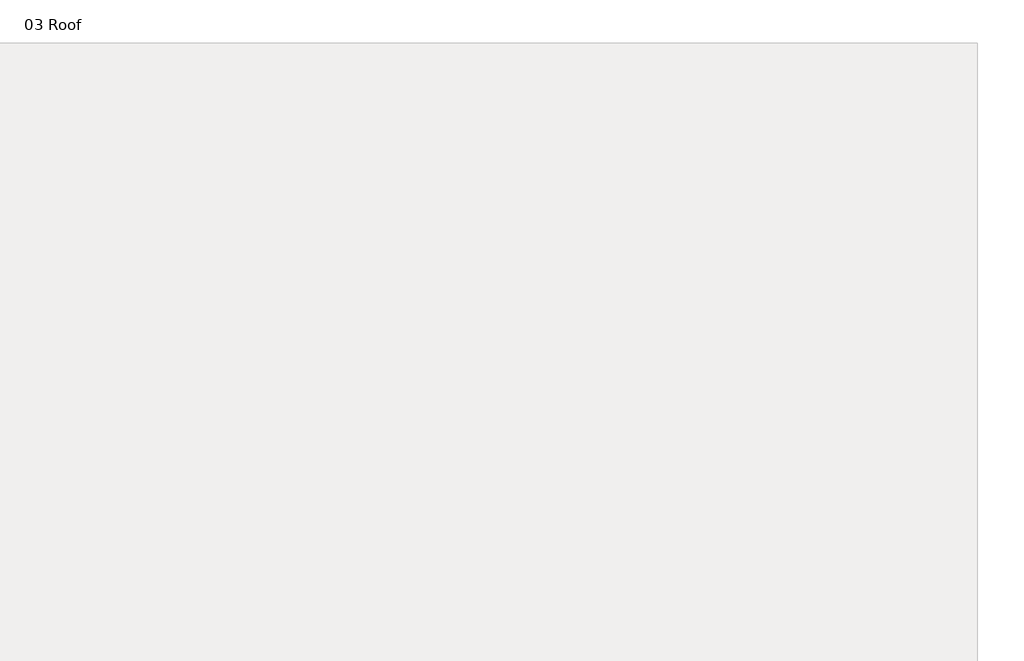
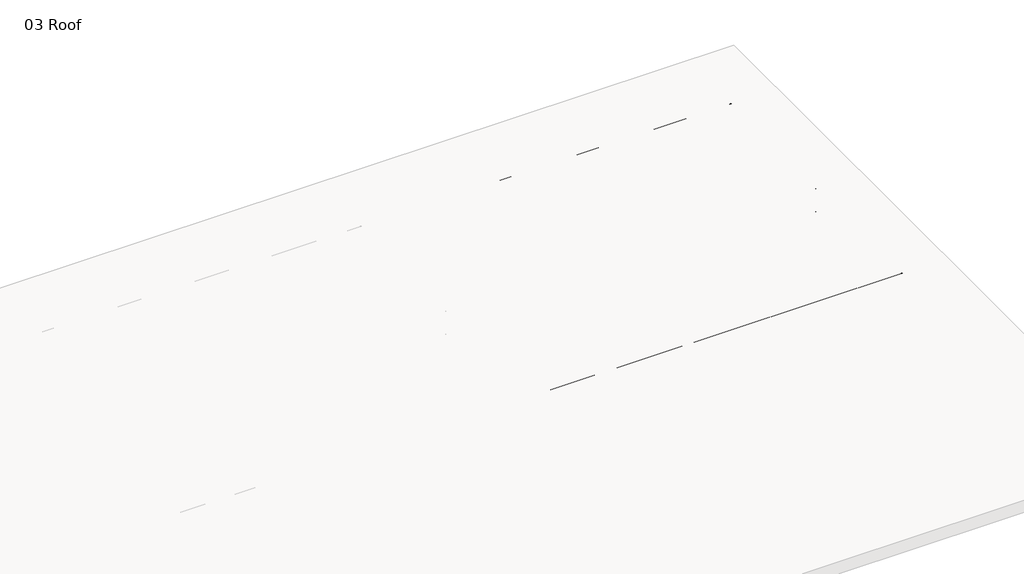
# One storey, part 4 of 4: 102 beams.
"""IFC4 building model written with IfcOpenShell, lengths in millimetres."""

import ifcopenshell
import ifcopenshell.guid

model = None  # the IFC model being written
_history = None  # IfcOwnerHistory: only IFC2X3 demands one
_inside = {}  # id of a spatial element -> (the spatial element, [elements in it])
_under = {}  # id of a project, library or spatial element -> (it, [spatial elements below it])
_declared = {}  # id of a project -> (the project, [libraries it declares])
_typed = {}  # id of a type object -> (the type object, [elements of that type])
_made_of = {}  # id of a material, layer set ... -> (it, [elements and type objects made of it])


def new_model(schema):
    """Start an empty IFC model of exactly this schema.

    Asked for "IFC4X3", IfcOpenShell would pick the latest addendum, in which some entities
    have other attributes; the version numbers below select the first issue.
    IFC2X3 requires an IfcOwnerHistory on every rooted entity: one is made here for all.
    """
    global model, _history
    if schema == "IFC4X3":
        model = ifcopenshell.file(schema_version=(4, 3, 0, 0))
    else:
        model = ifcopenshell.file(schema=schema)
    _inside.clear()
    _under.clear()
    _declared.clear()
    _typed.clear()
    _made_of.clear()
    _history = None
    if model.schema == "IFC2X3":
        org = make("IfcOrganization", Name="unknown")
        user = make(
            "IfcPersonAndOrganization",
            ThePerson=make("IfcPerson", FamilyName="unknown"),
            TheOrganization=org,
        )
        app = make(
            "IfcApplication",
            ApplicationDeveloper=org,
            Version="unknown",
            ApplicationFullName="unknown",
            ApplicationIdentifier="unknown",
        )
        _history = make(
            "IfcOwnerHistory",
            OwningUser=user,
            OwningApplication=app,
            ChangeAction="ADDED",
            CreationDate=0,
        )
    return model


def make(cls, **values):
    """One entity of the class cls with the attributes given. An attribute that is None is left unset."""
    return model.create_entity(
        cls, **{name: value for name, value in values.items() if value is not None}
    )


def rooted(cls, **values):
    """An entity with a GlobalId (a new one), such as an element, a storey or a relation."""
    return make(cls, GlobalId=ifcopenshell.guid.new(), OwnerHistory=_history, **values)


def si_unit(unit_type, name, prefix=None):
    """IfcSIUnit, for example si_unit("LENGTHUNIT", "METRE", prefix="MILLI")."""
    return make("IfcSIUnit", UnitType=unit_type, Prefix=prefix, Name=name)


def assignment(units):
    """IfcUnitAssignment: the units of a project."""
    return None if units is None else make("IfcUnitAssignment", Units=units)


def point(xyz):
    """IfcCartesianPoint."""
    return None if xyz is None else make("IfcCartesianPoint", Coordinates=xyz)


def direction(xyz):
    """IfcDirection."""
    return None if xyz is None else make("IfcDirection", DirectionRatios=xyz)


def frame(location, z_axis=None, x_axis=None):
    """IfcAxis2Placement3D, a coordinate frame: its origin and axes. An axis left out is left unset."""
    return make(
        "IfcAxis2Placement3D",
        Location=point(location),
        Axis=direction(z_axis),
        RefDirection=direction(x_axis),
    )


def frame_2d(location, x_axis=None):
    """IfcAxis2Placement2D, a coordinate frame in the plane: its origin and x axis."""
    return make(
        "IfcAxis2Placement2D", Location=point(location), RefDirection=direction(x_axis)
    )


def origin():
    """The frame at (0, 0, 0) with its axes left unset."""
    return frame((0.0, 0.0, 0.0))


def place(relative_to, where):
    """IfcLocalPlacement: puts the frame where relative to a parent placement (None: the world)."""
    return make(
        "IfcLocalPlacement", PlacementRelTo=relative_to, RelativePlacement=where
    )


def context(
    kind, dimensions, precision=None, world=None, true_north=None, identifier=None
):
    """IfcGeometricRepresentationContext, for example the 3D "Model" context."""
    return make(
        "IfcGeometricRepresentationContext",
        ContextIdentifier=identifier,
        ContextType=kind,
        CoordinateSpaceDimension=dimensions,
        Precision=precision,
        WorldCoordinateSystem=world,
        TrueNorth=true_north,
    )


def project(units=None, contexts=None):
    """IfcProject with its units and contexts."""
    return rooted(
        "IfcProject",
        Name="project",
        RepresentationContexts=contexts,
        UnitsInContext=assignment(units),
    )


def spatial(cls, under=None, at=None, **own):
    """A site, building, storey or space (cls), placed at a placement, below another one or the project."""
    s = rooted(cls, ObjectPlacement=at, **own)
    if under is not None:
        _under.setdefault(under.id(), (under, []))[1].append(s)
    return s


def polyline(points):
    """IfcPolyline through the points."""
    return make("IfcPolyline", Points=[point(p) for p in points])


def circle_curve(where, radius):
    """IfcCircle in the frame where."""
    return make("IfcCircle", Position=where, Radius=radius)


def trimmed(basis, trim1, trim2, sense, master):
    """IfcTrimmedCurve: the piece of a basis curve between two trims."""
    return make(
        "IfcTrimmedCurve",
        BasisCurve=basis,
        Trim1=trim1,
        Trim2=trim2,
        SenseAgreement=sense,
        MasterRepresentation=master,
    )


def segment(curve, same_sense, transition):
    """IfcCompositeCurveSegment."""
    return make(
        "IfcCompositeCurveSegment",
        Transition=transition,
        SameSense=same_sense,
        ParentCurve=curve,
    )


def composite_curve(segments, self_intersect=None):
    """IfcCompositeCurve: segments joined end to end."""
    return make("IfcCompositeCurve", Segments=segments, SelfIntersect=self_intersect)


def outline(outer, holes=None, kind="AREA"):
    """IfcArbitraryClosedProfileDef: a profile drawn as a closed curve; with holes, ...WithVoids."""
    if holes is None:
        return make("IfcArbitraryClosedProfileDef", ProfileType=kind, OuterCurve=outer)
    return make(
        "IfcArbitraryProfileDefWithVoids",
        ProfileType=kind,
        OuterCurve=outer,
        InnerCurves=holes,
    )


def extrude(swept, where, along, depth):
    """IfcExtrudedAreaSolid: the profile swept, set in the frame where, extruded along a direction by depth."""
    return make(
        "IfcExtrudedAreaSolid",
        SweptArea=swept,
        Position=where,
        ExtrudedDirection=direction(along),
        Depth=depth,
    )


def shape(context_of_items, identifier, shape_type, items):
    """IfcShapeRepresentation: the items that make up one representation, for example the "Body"."""
    return make(
        "IfcShapeRepresentation",
        ContextOfItems=context_of_items,
        RepresentationIdentifier=identifier,
        RepresentationType=shape_type,
        Items=items,
    )


def source(mapping_origin, context_of_items, identifier, shape_type, items):
    """IfcRepresentationMap: a shape defined once, which mapped items show again and again."""
    return make(
        "IfcRepresentationMap",
        MappingOrigin=mapping_origin,
        MappedRepresentation=shape(context_of_items, identifier, shape_type, items),
    )


def transform(
    local_origin,
    x_axis=None,
    y_axis=None,
    z_axis=None,
    scale=None,
    scale2=None,
    scale3=None,
    uniform=True,
):
    """IfcCartesianTransformationOperator3D, or its non-uniform kind. x_axis, y_axis, z_axis: its Axis1, 2, 3."""
    if uniform:
        return make(
            "IfcCartesianTransformationOperator3D",
            Axis1=direction(x_axis),
            Axis2=direction(y_axis),
            LocalOrigin=point(local_origin),
            Scale=scale,
            Axis3=direction(z_axis),
        )
    return make(
        "IfcCartesianTransformationOperator3DnonUniform",
        Axis1=direction(x_axis),
        Axis2=direction(y_axis),
        LocalOrigin=point(local_origin),
        Scale=scale,
        Axis3=direction(z_axis),
        Scale2=scale2,
        Scale3=scale3,
    )


def mapped(mapping_source, mapping_target):
    """IfcMappedItem: shows the shape of a source again, moved by a transform."""
    return make(
        "IfcMappedItem", MappingSource=mapping_source, MappingTarget=mapping_target
    )


def made_of(thing, what):
    """Note that an element or type object is made of a material, layer set ...; save() writes the relation."""
    if what is not None:
        _made_of.setdefault(what.id(), (what, []))[1].append(thing)
    return thing


def element(
    cls,
    number,
    at=None,
    inside=None,
    cuts=None,
    type_object=None,
    material=None,
    context=None,
    identifier="Body",
    shape_type=None,
    held_by="IfcProductDefinitionShape",
    body=None,
    shapes=None,
    **own,
):
    """One element of the class cls, such as IfcWall. Its Tag is "e" and its number.

    at: its placement. inside: the storey or other place that contains it. cuts: it is an
    opening in that element (IfcRelVoidsElement). A single representation is given by context,
    identifier, shape_type and body (its items); several are given by shapes. held_by: the class
    of the entity that holds the representations. save() writes the other relations.
    """
    e = rooted(cls, Tag="e%d" % number, ObjectPlacement=at, **own)
    if body is not None:
        shapes = [shape(context, identifier, shape_type, body)]
    if shapes is not None:
        e.Representation = make(held_by, Representations=shapes)
    if inside is not None:
        _inside.setdefault(inside.id(), (inside, []))[1].append(e)
    if cuts is not None:
        rooted(
            "IfcRelVoidsElement", RelatingBuildingElement=cuts, RelatedOpeningElement=e
        )
    if type_object is not None:
        _typed.setdefault(type_object.id(), (type_object, []))[1].append(e)
    return made_of(e, material)


def aggregate(whole, parts):
    """IfcRelAggregates: a whole, such as a stair, and the parts it consists of."""
    return rooted("IfcRelAggregates", RelatingObject=whole, RelatedObjects=parts)


def save(model, path):
    """Write the relations noted so far, then the file.

    IfcRelAggregates (storeys below a building ...), IfcRelContainedInSpatialStructure (elements
    in a storey), IfcRelDefinesByType, IfcRelAssociatesMaterial and IfcRelDeclares: one each for
    every whole, place, type object, material and project.
    """
    for whole, parts in _under.values():
        aggregate(whole, parts)
    for where, things in _inside.values():
        rooted(
            "IfcRelContainedInSpatialStructure",
            RelatedElements=things,
            RelatingStructure=where,
        )
    for kind, things in _typed.values():
        rooted("IfcRelDefinesByType", RelatedObjects=things, RelatingType=kind)
    for what, things in _made_of.values():
        rooted("IfcRelAssociatesMaterial", RelatedObjects=things, RelatingMaterial=what)
    for by, libraries in _declared.values():
        rooted("IfcRelDeclares", RelatingContext=by, RelatedDefinitions=libraries)
    model.write(path)


def ub_universal_beam_305x165x40ub_24de31be(model_context):
    return source(origin(), model_context, "Body", "SweptSolid", [
        extrude(outline(composite_curve([segment(polyline([(82.5, -141.5), (82.5, -151.7), (-82.5, -151.7), (-82.5, -141.5), (-11.9, -141.5)]), True, "CONTINUOUS"), segment(trimmed(circle_curve(frame_2d((-11.9, -132.6)), 8.9), [point((-11.9, -141.5))], [point((-3.0, -132.6))], True, "CARTESIAN"), True, "CONTINUOUS"), segment(polyline([(-3.0, -132.6), (-3.0, 132.6)]), True, "CONTINUOUS"), segment(trimmed(circle_curve(frame_2d((-11.9, 132.6)), 8.9), [point((-3.0, 132.6))], [point((-11.9, 141.5))], True, "CARTESIAN"), True, "CONTINUOUS"), segment(polyline([(-11.9, 141.5), (-82.5, 141.5), (-82.5, 151.7), (82.5, 151.7), (82.5, 141.5), (11.9, 141.5)]), True, "CONTINUOUS"), segment(trimmed(circle_curve(frame_2d((11.9, 132.6)), 8.9), [point((11.9, 141.5))], [point((3.0, 132.6))], True, "CARTESIAN"), True, "CONTINUOUS"), segment(polyline([(3.0, 132.6), (3.0, -132.6)]), True, "CONTINUOUS"), segment(trimmed(circle_curve(frame_2d((11.9, -132.6)), 8.9), [point((3.0, -132.6))], [point((11.9, -141.5))], True, "CARTESIAN"), True, "CONTINUOUS"), segment(polyline([(11.9, -141.5), (82.5, -141.5)]), True, "CONTINUOUS")], self_intersect=False)), frame((-335.6, 0.0, 0.0), z_axis=(1.0, 0.0, 0.0), x_axis=(0.0, 1.0, 0.0)), (0.0, 0.0, 1.0), 671.2),
    ])


def ub_universal_beam_305x165x40ub_f67fc52f(model_context):
    return source(origin(), model_context, "Body", "SweptSolid", [
        extrude(outline(composite_curve([segment(polyline([(82.5, -141.5), (82.5, -151.7), (-82.5, -151.7), (-82.5, -141.5), (-11.9, -141.5)]), True, "CONTINUOUS"), segment(trimmed(circle_curve(frame_2d((-11.9, -132.6)), 8.9), [point((-11.9, -141.5))], [point((-3.0, -132.6))], True, "CARTESIAN"), True, "CONTINUOUS"), segment(polyline([(-3.0, -132.6), (-3.0, 132.6)]), True, "CONTINUOUS"), segment(trimmed(circle_curve(frame_2d((-11.9, 132.6)), 8.9), [point((-3.0, 132.6))], [point((-11.9, 141.5))], True, "CARTESIAN"), True, "CONTINUOUS"), segment(polyline([(-11.9, 141.5), (-82.5, 141.5), (-82.5, 151.7), (82.5, 151.7), (82.5, 141.5), (11.9, 141.5)]), True, "CONTINUOUS"), segment(trimmed(circle_curve(frame_2d((11.9, 132.6)), 8.9), [point((11.9, 141.5))], [point((3.0, 132.6))], True, "CARTESIAN"), True, "CONTINUOUS"), segment(polyline([(3.0, 132.6), (3.0, -132.6)]), True, "CONTINUOUS"), segment(trimmed(circle_curve(frame_2d((11.9, -132.6)), 8.9), [point((3.0, -132.6))], [point((11.9, -141.5))], True, "CARTESIAN"), True, "CONTINUOUS"), segment(polyline([(11.9, -141.5), (82.5, -141.5)]), True, "CONTINUOUS")], self_intersect=False)), frame((-7125.0, 0.0, 0.0), z_axis=(1.0, 0.0, 0.0), x_axis=(0.0, 1.0, 0.0)), (0.0, 0.0, 1.0), 14250.0),
    ])


def ub_universal_beam_305x165x40ub_26fb8d3a(model_context):
    return source(origin(), model_context, "Body", "SweptSolid", [
        extrude(outline(composite_curve([segment(polyline([(82.5, -141.5), (82.5, -151.7), (-82.5, -151.7), (-82.5, -141.5), (-11.9, -141.5)]), True, "CONTINUOUS"), segment(trimmed(circle_curve(frame_2d((-11.9, -132.6)), 8.9), [point((-11.9, -141.5))], [point((-3.0, -132.6))], True, "CARTESIAN"), True, "CONTINUOUS"), segment(polyline([(-3.0, -132.6), (-3.0, 132.6)]), True, "CONTINUOUS"), segment(trimmed(circle_curve(frame_2d((-11.9, 132.6)), 8.9), [point((-3.0, 132.6))], [point((-11.9, 141.5))], True, "CARTESIAN"), True, "CONTINUOUS"), segment(polyline([(-11.9, 141.5), (-82.5, 141.5), (-82.5, 151.7), (82.5, 151.7), (82.5, 141.5), (11.9, 141.5)]), True, "CONTINUOUS"), segment(trimmed(circle_curve(frame_2d((11.9, 132.6)), 8.9), [point((11.9, 141.5))], [point((3.0, 132.6))], True, "CARTESIAN"), True, "CONTINUOUS"), segment(polyline([(3.0, 132.6), (3.0, -132.6)]), True, "CONTINUOUS"), segment(trimmed(circle_curve(frame_2d((11.9, -132.6)), 8.9), [point((3.0, -132.6))], [point((11.9, -141.5))], True, "CARTESIAN"), True, "CONTINUOUS"), segment(polyline([(11.9, -141.5), (82.5, -141.5)]), True, "CONTINUOUS")], self_intersect=False)), frame((-347.8807825, 0.0, 0.0), z_axis=(1.0, 0.0, 0.0), x_axis=(0.0, 1.0, 0.0)), (0.0, 0.0, 1.0), 695.761565),
    ])


model = new_model("IFC4")

# Units and contexts
model_context = context("Model", 3, world=origin())
ifc_project = project(units=[si_unit("LENGTHUNIT", "METRE", prefix="MILLI")], contexts=[model_context])

# Site, building, storey
site = spatial("IfcSite", under=ifc_project)
building = spatial("IfcBuilding", under=site)
storey = spatial("IfcBuildingStorey", under=building, Name="03 Roof", Elevation=8000.0)

# Beams
placement = place(None, origin())
ub_universal_beam_305x165x40ub_shape = ub_universal_beam_305x165x40ub_24de31be(model_context)
element("IfcBeam", 1, ObjectType="UB-Universal Beam : 305x165x40UB", at=placement, inside=storey, context=model_context, shape_type="MappedRepresentation", body=[
    mapped(ub_universal_beam_305x165x40ub_shape, transform((5723.4493174, 12261.9474871, 7500.0), x_axis=(0.0, 0.0, 1.0), y_axis=(0.0, -1.0, 0.0), z_axis=(1.0, 0.0, 0.0))),
])
element("IfcBeam", 2, ObjectType="UB-Universal Beam : 305x165x40UB", at=placement, inside=storey, context=model_context, shape_type="MappedRepresentation", body=[
    mapped(ub_universal_beam_305x165x40ub_shape, transform((4535.9493174, 12261.9474871, 7500.0), x_axis=(0.0, 0.0, 1.0), y_axis=(0.0, -1.0, 0.0), z_axis=(1.0, 0.0, 0.0))),
])
element("IfcBeam", 3, ObjectType="UB-Universal Beam : 305x165x40UB", at=placement, inside=storey, context=model_context, shape_type="MappedRepresentation", body=[
    mapped(ub_universal_beam_305x165x40ub_shape, transform((3348.4493174, 12261.9474871, 7500.0), x_axis=(0.0, 0.0, 1.0), y_axis=(0.0, -1.0, 0.0), z_axis=(1.0, 0.0, 0.0))),
])
element("IfcBeam", 4, ObjectType="UB-Universal Beam : 305x165x40UB", at=placement, inside=storey, context=model_context, shape_type="MappedRepresentation", body=[
    mapped(ub_universal_beam_305x165x40ub_shape, transform((2160.9493174, 12261.9474871, 7500.0), x_axis=(0.0, 0.0, 1.0), y_axis=(0.0, -1.0, 0.0), z_axis=(1.0, 0.0, 0.0))),
])
element("IfcBeam", 5, ObjectType="UB-Universal Beam : 305x165x40UB", at=placement, inside=storey, context=model_context, shape_type="MappedRepresentation", body=[
    mapped(ub_universal_beam_305x165x40ub_shape, transform((6910.9493174, 12261.9474871, 7500.0), x_axis=(0.0, 0.0, 1.0), y_axis=(0.0, -1.0, 0.0), z_axis=(1.0, 0.0, 0.0))),
])
element("IfcBeam", 6, ObjectType="UB-Universal Beam : 305x165x40UB", at=placement, inside=storey, context=model_context, shape_type="MappedRepresentation", body=[
    mapped(ub_universal_beam_305x165x40ub_shape, transform((973.4493174, 12261.9474871, 7500.0), x_axis=(0.0, 0.0, 1.0), y_axis=(0.0, -1.0, 0.0), z_axis=(1.0, 0.0, 0.0))),
])
element("IfcBeam", 7, ObjectType="UB-Universal Beam : 305x165x40UB", at=placement, inside=storey, context=model_context, shape_type="MappedRepresentation", body=[
    mapped(ub_universal_beam_305x165x40ub_shape, transform((20723.4493174, 12261.9474871, 7500.0), x_axis=(0.0, 0.0, 1.0), y_axis=(0.0, -1.0, 0.0), z_axis=(1.0, 0.0, 0.0))),
])
element("IfcBeam", 8, ObjectType="UB-Universal Beam : 305x165x40UB", at=placement, inside=storey, context=model_context, shape_type="MappedRepresentation", body=[
    mapped(ub_universal_beam_305x165x40ub_shape, transform((8848.4493174, 12261.9474871, 7500.0), x_axis=(0.0, 0.0, 1.0), y_axis=(0.0, -1.0, 0.0), z_axis=(1.0, 0.0, 0.0))),
])
element("IfcBeam", 9, ObjectType="UB-Universal Beam : 305x165x40UB", at=placement, inside=storey, context=model_context, shape_type="MappedRepresentation", body=[
    mapped(ub_universal_beam_305x165x40ub_shape, transform((19535.9493174, 12261.9474871, 7500.0), x_axis=(0.0, 0.0, 1.0), y_axis=(0.0, -1.0, 0.0), z_axis=(1.0, 0.0, 0.0))),
])
element("IfcBeam", 10, ObjectType="UB-Universal Beam : 305x165x40UB", at=placement, inside=storey, context=model_context, shape_type="MappedRepresentation", body=[
    mapped(ub_universal_beam_305x165x40ub_shape, transform((10035.9493174, 12261.9474871, 7500.0), x_axis=(0.0, 0.0, 1.0), y_axis=(0.0, -1.0, 0.0), z_axis=(1.0, 0.0, 0.0))),
])
element("IfcBeam", 11, ObjectType="UB-Universal Beam : 305x165x40UB", at=placement, inside=storey, context=model_context, shape_type="MappedRepresentation", body=[
    mapped(ub_universal_beam_305x165x40ub_shape, transform((18348.4493174, 12261.9474871, 7500.0), x_axis=(0.0, 0.0, 1.0), y_axis=(0.0, -1.0, 0.0), z_axis=(1.0, 0.0, 0.0))),
])
element("IfcBeam", 12, ObjectType="UB-Universal Beam : 305x165x40UB", at=placement, inside=storey, context=model_context, shape_type="MappedRepresentation", body=[
    mapped(ub_universal_beam_305x165x40ub_shape, transform((17160.9493174, 12261.9474871, 7500.0), x_axis=(0.0, 0.0, 1.0), y_axis=(0.0, -1.0, 0.0), z_axis=(1.0, 0.0, 0.0))),
])
element("IfcBeam", 13, ObjectType="UB-Universal Beam : 305x165x40UB", at=placement, inside=storey, context=model_context, shape_type="MappedRepresentation", body=[
    mapped(ub_universal_beam_305x165x40ub_shape, transform((21910.9493174, 12261.9474871, 7500.0), x_axis=(0.0, 0.0, 1.0), y_axis=(0.0, -1.0, 0.0), z_axis=(1.0, 0.0, 0.0))),
])
element("IfcBeam", 14, ObjectType="UB-Universal Beam : 305x165x40UB", at=placement, inside=storey, context=model_context, shape_type="MappedRepresentation", body=[
    mapped(ub_universal_beam_305x165x40ub_shape, transform((15973.4493174, 12261.9474871, 7500.0), x_axis=(0.0, 0.0, 1.0), y_axis=(0.0, -1.0, 0.0), z_axis=(1.0, 0.0, 0.0))),
])
element("IfcBeam", 15, ObjectType="UB-Universal Beam : 305x165x40UB", at=placement, inside=storey, context=model_context, shape_type="MappedRepresentation", body=[
    mapped(ub_universal_beam_305x165x40ub_shape, transform((11223.4493174, 12261.9474871, 7500.0), x_axis=(0.0, 0.0, 1.0), y_axis=(0.0, -1.0, 0.0), z_axis=(1.0, 0.0, 0.0))),
])
element("IfcBeam", 16, ObjectType="UB-Universal Beam : 305x165x40UB", at=placement, inside=storey, context=model_context, shape_type="MappedRepresentation", body=[
    mapped(ub_universal_beam_305x165x40ub_shape, transform((12410.9493174, 12261.9474871, 7500.0), x_axis=(0.0, 0.0, 1.0), y_axis=(0.0, -1.0, 0.0), z_axis=(1.0, 0.0, 0.0))),
])
element("IfcBeam", 17, ObjectType="UB-Universal Beam : 305x165x40UB", at=placement, inside=storey, context=model_context, shape_type="MappedRepresentation", body=[
    mapped(ub_universal_beam_305x165x40ub_shape, transform((7660.9493174, 12261.9474871, 7500.0), x_axis=(0.0, 0.0, 1.0), y_axis=(0.0, -1.0, 0.0), z_axis=(1.0, 0.0, 0.0))),
])
element("IfcBeam", 18, ObjectType="UB-Universal Beam : 305x165x40UB", at=placement, inside=storey, context=model_context, shape_type="MappedRepresentation", body=[
    mapped(ub_universal_beam_305x165x40ub_shape, transform((13598.4493174, 12261.9474871, 7500.0), x_axis=(0.0, 0.0, 1.0), y_axis=(0.0, -1.0, 0.0), z_axis=(1.0, 0.0, 0.0))),
])
element("IfcBeam", 19, ObjectType="UB-Universal Beam : 305x165x40UB", at=placement, inside=storey, context=model_context, shape_type="MappedRepresentation", body=[
    mapped(ub_universal_beam_305x165x40ub_shape, transform((14785.9493174, 12261.9474871, 7500.0), x_axis=(0.0, 0.0, 1.0), y_axis=(0.0, -1.0, 0.0), z_axis=(1.0, 0.0, 0.0))),
])
element("IfcBeam", 20, ObjectType="UB-Universal Beam : 305x165x40UB", at=placement, inside=storey, context=model_context, shape_type="MappedRepresentation", body=[
    mapped(ub_universal_beam_305x165x40ub_shape, transform((5723.4493174, 6271.8474871, 7500.0), x_axis=(0.0, 0.0, 1.0), y_axis=(0.0, -1.0, 0.0), z_axis=(1.0, 0.0, 0.0))),
])
element("IfcBeam", 21, ObjectType="UB-Universal Beam : 305x165x40UB", at=placement, inside=storey, context=model_context, shape_type="MappedRepresentation", body=[
    mapped(ub_universal_beam_305x165x40ub_shape, transform((4535.9493174, 6271.8474871, 7500.0), x_axis=(0.0, 0.0, 1.0), y_axis=(0.0, -1.0, 0.0), z_axis=(1.0, 0.0, 0.0))),
])
element("IfcBeam", 22, ObjectType="UB-Universal Beam : 305x165x40UB", at=placement, inside=storey, context=model_context, shape_type="MappedRepresentation", body=[
    mapped(ub_universal_beam_305x165x40ub_shape, transform((3348.4493174, 6271.8474871, 7500.0), x_axis=(0.0, 0.0, 1.0), y_axis=(0.0, -1.0, 0.0), z_axis=(1.0, 0.0, 0.0))),
])
element("IfcBeam", 23, ObjectType="UB-Universal Beam : 305x165x40UB", at=placement, inside=storey, context=model_context, shape_type="MappedRepresentation", body=[
    mapped(ub_universal_beam_305x165x40ub_shape, transform((2160.9493174, 6271.8474871, 7500.0), x_axis=(0.0, 0.0, 1.0), y_axis=(0.0, -1.0, 0.0), z_axis=(1.0, 0.0, 0.0))),
])
element("IfcBeam", 24, ObjectType="UB-Universal Beam : 305x165x40UB", at=placement, inside=storey, context=model_context, shape_type="MappedRepresentation", body=[
    mapped(ub_universal_beam_305x165x40ub_shape, transform((6910.9493174, 6271.8474871, 7500.0), x_axis=(0.0, 0.0, 1.0), y_axis=(0.0, -1.0, 0.0), z_axis=(1.0, 0.0, 0.0))),
])
element("IfcBeam", 25, ObjectType="UB-Universal Beam : 305x165x40UB", at=placement, inside=storey, context=model_context, shape_type="MappedRepresentation", body=[
    mapped(ub_universal_beam_305x165x40ub_shape, transform((20723.4493174, 6271.8474871, 7500.0), x_axis=(0.0, 0.0, 1.0), y_axis=(0.0, -1.0, 0.0), z_axis=(1.0, 0.0, 0.0))),
])
element("IfcBeam", 26, ObjectType="UB-Universal Beam : 305x165x40UB", at=placement, inside=storey, context=model_context, shape_type="MappedRepresentation", body=[
    mapped(ub_universal_beam_305x165x40ub_shape, transform((8848.4493174, 6271.8474871, 7500.0), x_axis=(0.0, 0.0, 1.0), y_axis=(0.0, -1.0, 0.0), z_axis=(1.0, 0.0, 0.0))),
])
element("IfcBeam", 27, ObjectType="UB-Universal Beam : 305x165x40UB", at=placement, inside=storey, context=model_context, shape_type="MappedRepresentation", body=[
    mapped(ub_universal_beam_305x165x40ub_shape, transform((19535.9493174, 6271.8474871, 7500.0), x_axis=(0.0, 0.0, 1.0), y_axis=(0.0, -1.0, 0.0), z_axis=(1.0, 0.0, 0.0))),
])
element("IfcBeam", 28, ObjectType="UB-Universal Beam : 305x165x40UB", at=placement, inside=storey, context=model_context, shape_type="MappedRepresentation", body=[
    mapped(ub_universal_beam_305x165x40ub_shape, transform((10035.9493174, 6271.8474871, 7500.0), x_axis=(0.0, 0.0, 1.0), y_axis=(0.0, -1.0, 0.0), z_axis=(1.0, 0.0, 0.0))),
])
element("IfcBeam", 29, ObjectType="UB-Universal Beam : 305x165x40UB", at=placement, inside=storey, context=model_context, shape_type="MappedRepresentation", body=[
    mapped(ub_universal_beam_305x165x40ub_shape, transform((18348.4493174, 6271.8474871, 7500.0), x_axis=(0.0, 0.0, 1.0), y_axis=(0.0, -1.0, 0.0), z_axis=(1.0, 0.0, 0.0))),
])
element("IfcBeam", 30, ObjectType="UB-Universal Beam : 305x165x40UB", at=placement, inside=storey, context=model_context, shape_type="MappedRepresentation", body=[
    mapped(ub_universal_beam_305x165x40ub_shape, transform((17160.9493174, 6271.8474871, 7500.0), x_axis=(0.0, 0.0, 1.0), y_axis=(0.0, -1.0, 0.0), z_axis=(1.0, 0.0, 0.0))),
])
element("IfcBeam", 31, ObjectType="UB-Universal Beam : 305x165x40UB", at=placement, inside=storey, context=model_context, shape_type="MappedRepresentation", body=[
    mapped(ub_universal_beam_305x165x40ub_shape, transform((21910.9493174, 6271.8474871, 7500.0), x_axis=(0.0, 0.0, 1.0), y_axis=(0.0, -1.0, 0.0), z_axis=(1.0, 0.0, 0.0))),
])
element("IfcBeam", 32, ObjectType="UB-Universal Beam : 305x165x40UB", at=placement, inside=storey, context=model_context, shape_type="MappedRepresentation", body=[
    mapped(ub_universal_beam_305x165x40ub_shape, transform((15973.4493174, 6271.8474871, 7500.0), x_axis=(0.0, 0.0, 1.0), y_axis=(0.0, -1.0, 0.0), z_axis=(1.0, 0.0, 0.0))),
])
element("IfcBeam", 33, ObjectType="UB-Universal Beam : 305x165x40UB", at=placement, inside=storey, context=model_context, shape_type="MappedRepresentation", body=[
    mapped(ub_universal_beam_305x165x40ub_shape, transform((11223.4493174, 6271.8474871, 7500.0), x_axis=(0.0, 0.0, 1.0), y_axis=(0.0, -1.0, 0.0), z_axis=(1.0, 0.0, 0.0))),
])
element("IfcBeam", 34, ObjectType="UB-Universal Beam : 305x165x40UB", at=placement, inside=storey, context=model_context, shape_type="MappedRepresentation", body=[
    mapped(ub_universal_beam_305x165x40ub_shape, transform((12410.9493174, 6271.8474871, 7500.0), x_axis=(0.0, 0.0, 1.0), y_axis=(0.0, -1.0, 0.0), z_axis=(1.0, 0.0, 0.0))),
])
element("IfcBeam", 35, ObjectType="UB-Universal Beam : 305x165x40UB", at=placement, inside=storey, context=model_context, shape_type="MappedRepresentation", body=[
    mapped(ub_universal_beam_305x165x40ub_shape, transform((7660.9493174, 6271.8474871, 7500.0), x_axis=(0.0, 0.0, 1.0), y_axis=(0.0, -1.0, 0.0), z_axis=(1.0, 0.0, 0.0))),
])
element("IfcBeam", 36, ObjectType="UB-Universal Beam : 305x165x40UB", at=placement, inside=storey, context=model_context, shape_type="MappedRepresentation", body=[
    mapped(ub_universal_beam_305x165x40ub_shape, transform((13598.4493174, 6271.8474871, 7500.0), x_axis=(0.0, 0.0, 1.0), y_axis=(0.0, -1.0, 0.0), z_axis=(1.0, 0.0, 0.0))),
])
element("IfcBeam", 37, ObjectType="UB-Universal Beam : 305x165x40UB", at=placement, inside=storey, context=model_context, shape_type="MappedRepresentation", body=[
    mapped(ub_universal_beam_305x165x40ub_shape, transform((14785.9493174, 6271.8474871, 7500.0), x_axis=(0.0, 0.0, 1.0), y_axis=(0.0, -1.0, 0.0), z_axis=(1.0, 0.0, 0.0))),
])
element("IfcBeam", 38, ObjectType="UB-Universal Beam : 305x165x40UB", at=placement, inside=storey, context=model_context, shape_type="MappedRepresentation", body=[
    mapped(ub_universal_beam_305x165x40ub_shape, transform((20723.4493174, 271.8474871, 7500.0), x_axis=(0.0, 0.0, 1.0), y_axis=(0.0, -1.0, 0.0), z_axis=(1.0, 0.0, 0.0))),
])
element("IfcBeam", 39, ObjectType="UB-Universal Beam : 305x165x40UB", at=placement, inside=storey, context=model_context, shape_type="MappedRepresentation", body=[
    mapped(ub_universal_beam_305x165x40ub_shape, transform((8848.4493174, 271.8474871, 7500.0), x_axis=(0.0, 0.0, 1.0), y_axis=(0.0, -1.0, 0.0), z_axis=(1.0, 0.0, 0.0))),
])
element("IfcBeam", 40, ObjectType="UB-Universal Beam : 305x165x40UB", at=placement, inside=storey, context=model_context, shape_type="MappedRepresentation", body=[
    mapped(ub_universal_beam_305x165x40ub_shape, transform((19535.9493174, 271.8474871, 7500.0), x_axis=(0.0, 0.0, 1.0), y_axis=(0.0, -1.0, 0.0), z_axis=(1.0, 0.0, 0.0))),
])
element("IfcBeam", 41, ObjectType="UB-Universal Beam : 305x165x40UB", at=placement, inside=storey, context=model_context, shape_type="MappedRepresentation", body=[
    mapped(ub_universal_beam_305x165x40ub_shape, transform((10035.9493174, 271.8474871, 7500.0), x_axis=(0.0, 0.0, 1.0), y_axis=(0.0, -1.0, 0.0), z_axis=(1.0, 0.0, 0.0))),
])
element("IfcBeam", 42, ObjectType="UB-Universal Beam : 305x165x40UB", at=placement, inside=storey, context=model_context, shape_type="MappedRepresentation", body=[
    mapped(ub_universal_beam_305x165x40ub_shape, transform((18348.4493174, 271.8474871, 7500.0), x_axis=(0.0, 0.0, 1.0), y_axis=(0.0, -1.0, 0.0), z_axis=(1.0, 0.0, 0.0))),
])
element("IfcBeam", 43, ObjectType="UB-Universal Beam : 305x165x40UB", at=placement, inside=storey, context=model_context, shape_type="MappedRepresentation", body=[
    mapped(ub_universal_beam_305x165x40ub_shape, transform((17160.9493174, 271.8474871, 7500.0), x_axis=(0.0, 0.0, 1.0), y_axis=(0.0, -1.0, 0.0), z_axis=(1.0, 0.0, 0.0))),
])
element("IfcBeam", 44, ObjectType="UB-Universal Beam : 305x165x40UB", at=placement, inside=storey, context=model_context, shape_type="MappedRepresentation", body=[
    mapped(ub_universal_beam_305x165x40ub_shape, transform((21910.9493174, 271.8474871, 7500.0), x_axis=(0.0, 0.0, 1.0), y_axis=(0.0, -1.0, 0.0), z_axis=(1.0, 0.0, 0.0))),
])
element("IfcBeam", 45, ObjectType="UB-Universal Beam : 305x165x40UB", at=placement, inside=storey, context=model_context, shape_type="MappedRepresentation", body=[
    mapped(ub_universal_beam_305x165x40ub_shape, transform((15973.4493174, 271.8474871, 7500.0), x_axis=(0.0, 0.0, 1.0), y_axis=(0.0, -1.0, 0.0), z_axis=(1.0, 0.0, 0.0))),
])
element("IfcBeam", 46, ObjectType="UB-Universal Beam : 305x165x40UB", at=placement, inside=storey, context=model_context, shape_type="MappedRepresentation", body=[
    mapped(ub_universal_beam_305x165x40ub_shape, transform((11223.4493174, 271.8474871, 7500.0), x_axis=(0.0, 0.0, 1.0), y_axis=(0.0, -1.0, 0.0), z_axis=(1.0, 0.0, 0.0))),
])
element("IfcBeam", 47, ObjectType="UB-Universal Beam : 305x165x40UB", at=placement, inside=storey, context=model_context, shape_type="MappedRepresentation", body=[
    mapped(ub_universal_beam_305x165x40ub_shape, transform((12410.9493174, 271.8474871, 7500.0), x_axis=(0.0, 0.0, 1.0), y_axis=(0.0, -1.0, 0.0), z_axis=(1.0, 0.0, 0.0))),
])
element("IfcBeam", 48, ObjectType="UB-Universal Beam : 305x165x40UB", at=placement, inside=storey, context=model_context, shape_type="MappedRepresentation", body=[
    mapped(ub_universal_beam_305x165x40ub_shape, transform((13598.4493174, 271.8474871, 7500.0), x_axis=(0.0, 0.0, 1.0), y_axis=(0.0, -1.0, 0.0), z_axis=(1.0, 0.0, 0.0))),
])
element("IfcBeam", 49, ObjectType="UB-Universal Beam : 305x165x40UB", at=placement, inside=storey, context=model_context, shape_type="MappedRepresentation", body=[
    mapped(ub_universal_beam_305x165x40ub_shape, transform((14785.9493174, 271.8474871, 7500.0), x_axis=(0.0, 0.0, 1.0), y_axis=(0.0, -1.0, 0.0), z_axis=(1.0, 0.0, 0.0))),
])
ub_universal_beam_305x165x40ub_2_shape = ub_universal_beam_305x165x40ub_f67fc52f(model_context)
element("IfcBeam", 50, ObjectType="UB-Universal Beam : 305x165x40UB", at=placement, inside=storey, context=model_context, shape_type="MappedRepresentation", body=[
    mapped(ub_universal_beam_305x165x40ub_2_shape, transform((14785.9493174, 12261.9474871, 7000.0), x_axis=(1.0, 0.0, 0.0), y_axis=(0.0, 1.0, 0.0), z_axis=(0.0, 0.0, 1.0))),
])
element("IfcBeam", 51, ObjectType="UB-Universal Beam : 305x165x40UB", at=placement, inside=storey, context=model_context, shape_type="MappedRepresentation", body=[
    mapped(ub_universal_beam_305x165x40ub_2_shape, transform((14785.9493174, 12261.9474871, 8000.0), x_axis=(1.0, 0.0, 0.0), y_axis=(0.0, 1.0, 0.0), z_axis=(0.0, 0.0, 1.0))),
])
element("IfcBeam", 52, ObjectType="UB-Universal Beam : 305x165x40UB", at=placement, inside=storey, context=model_context, shape_type="MappedRepresentation", body=[
    mapped(ub_universal_beam_305x165x40ub_2_shape, transform((14785.9493174, 6271.8474871, 7000.0), x_axis=(1.0, 0.0, 0.0), y_axis=(0.0, 1.0, 0.0), z_axis=(0.0, 0.0, 1.0))),
])
element("IfcBeam", 53, ObjectType="UB-Universal Beam : 305x165x40UB", at=placement, inside=storey, context=model_context, shape_type="MappedRepresentation", body=[
    mapped(ub_universal_beam_305x165x40ub_2_shape, transform((14785.9493174, 6271.8474871, 8000.0), x_axis=(1.0, 0.0, 0.0), y_axis=(0.0, 1.0, 0.0), z_axis=(0.0, 0.0, 1.0))),
])
element("IfcBeam", 54, ObjectType="UB-Universal Beam : 305x165x40UB", at=placement, inside=storey, context=model_context, shape_type="MappedRepresentation", body=[
    mapped(ub_universal_beam_305x165x40ub_2_shape, transform((14785.9493174, 271.8474871, 7000.0), x_axis=(1.0, 0.0, 0.0), y_axis=(0.0, 1.0, 0.0), z_axis=(0.0, 0.0, 1.0))),
])
element("IfcBeam", 55, ObjectType="UB-Universal Beam : 305x165x40UB", at=placement, inside=storey, context=model_context, shape_type="MappedRepresentation", body=[
    mapped(ub_universal_beam_305x165x40ub_2_shape, transform((14785.9493174, 271.8474871, 8000.0), x_axis=(1.0, 0.0, 0.0), y_axis=(0.0, 1.0, 0.0), z_axis=(0.0, 0.0, 1.0))),
])
ub_universal_beam_305x165x40ub_3_shape = ub_universal_beam_305x165x40ub_26fb8d3a(model_context)
element("IfcBeam", 56, ObjectType="UB-Universal Beam : 305x165x40UB", at=placement, inside=storey, context=model_context, shape_type="MappedRepresentation", body=[
    mapped(ub_universal_beam_305x165x40ub_3_shape, transform((5129.6993174, 12261.9474871, 7500.0), x_axis=(0.764911198117045, 0.0, 0.6441357457827868), y_axis=(0.0, -1.0, 0.0), z_axis=(0.6441357457827868, 0.0, -0.764911198117045))),
])
element("IfcBeam", 57, ObjectType="UB-Universal Beam : 305x165x40UB", at=placement, inside=storey, context=model_context, shape_type="MappedRepresentation", body=[
    mapped(ub_universal_beam_305x165x40ub_3_shape, transform((3942.1993174, 12261.9474871, 7500.0), x_axis=(0.7649111981170463, 0.0, 0.6441357457827852), y_axis=(0.0, -1.0, 0.0), z_axis=(0.6441357457827852, 0.0, -0.7649111981170463))),
])
element("IfcBeam", 58, ObjectType="UB-Universal Beam : 305x165x40UB", at=placement, inside=storey, context=model_context, shape_type="MappedRepresentation", body=[
    mapped(ub_universal_beam_305x165x40ub_3_shape, transform((2754.6993174, 12261.9474871, 7500.0), x_axis=(0.7649111981170467, 0.0, 0.6441357457827848), y_axis=(0.0, -1.0, 0.0), z_axis=(0.6441357457827848, 0.0, -0.7649111981170467))),
])
element("IfcBeam", 59, ObjectType="UB-Universal Beam : 305x165x40UB", at=placement, inside=storey, context=model_context, shape_type="MappedRepresentation", body=[
    mapped(ub_universal_beam_305x165x40ub_3_shape, transform((1567.1993174, 12261.9474871, 7500.0), x_axis=(0.7649111981170473, 0.0, 0.6441357457827839), y_axis=(0.0, -1.0, 0.0), z_axis=(0.6441357457827839, 0.0, -0.7649111981170473))),
])
element("IfcBeam", 60, ObjectType="UB-Universal Beam : 305x165x40UB", at=placement, inside=storey, context=model_context, shape_type="MappedRepresentation", body=[
    mapped(ub_universal_beam_305x165x40ub_3_shape, transform((6317.1993174, 12261.9474871, 7500.0), x_axis=(0.7649111981170472, 0.0, 0.6441357457827841), y_axis=(0.0, -1.0, 0.0), z_axis=(0.6441357457827841, 0.0, -0.7649111981170472))),
])
element("IfcBeam", 61, ObjectType="UB-Universal Beam : 305x165x40UB", at=placement, inside=storey, context=model_context, shape_type="MappedRepresentation", body=[
    mapped(ub_universal_beam_305x165x40ub_3_shape, transform((379.6993174, 12261.9474871, 7500.0), x_axis=(0.764911198117048, 0.0, 0.6441357457827831), y_axis=(0.0, -1.0, 0.0), z_axis=(0.6441357457827831, 0.0, -0.764911198117048))),
])
element("IfcBeam", 62, ObjectType="UB-Universal Beam : 305x165x40UB", at=placement, inside=storey, context=model_context, shape_type="MappedRepresentation", body=[
    mapped(ub_universal_beam_305x165x40ub_3_shape, transform((20129.6993174, 12261.9474871, 7500.0), x_axis=(0.764911198117045, 0.0, 0.6441357457827868), y_axis=(0.0, -1.0, 0.0), z_axis=(0.6441357457827868, 0.0, -0.764911198117045))),
])
element("IfcBeam", 63, ObjectType="UB-Universal Beam : 305x165x40UB", at=placement, inside=storey, context=model_context, shape_type="MappedRepresentation", body=[
    mapped(ub_universal_beam_305x165x40ub_3_shape, transform((9442.1993174, 12261.9474871, 7500.0), x_axis=(0.7649111981170519, 0.0, -0.6441357457827785), y_axis=(0.0, -1.0, 0.0), z_axis=(-0.6441357457827785, 0.0, -0.7649111981170519))),
])
element("IfcBeam", 64, ObjectType="UB-Universal Beam : 305x165x40UB", at=placement, inside=storey, context=model_context, shape_type="MappedRepresentation", body=[
    mapped(ub_universal_beam_305x165x40ub_3_shape, transform((18942.1993174, 12261.9474871, 7500.0), x_axis=(0.7649111981170457, 0.0, 0.6441357457827859), y_axis=(0.0, -1.0, 0.0), z_axis=(0.6441357457827859, 0.0, -0.7649111981170457))),
])
element("IfcBeam", 65, ObjectType="UB-Universal Beam : 305x165x40UB", at=placement, inside=storey, context=model_context, shape_type="MappedRepresentation", body=[
    mapped(ub_universal_beam_305x165x40ub_3_shape, transform((10629.6993174, 12261.9474871, 7500.0), x_axis=(0.7649111981170518, 0.0, -0.6441357457827787), y_axis=(0.0, -1.0, 0.0), z_axis=(-0.6441357457827787, 0.0, -0.7649111981170518))),
])
element("IfcBeam", 66, ObjectType="UB-Universal Beam : 305x165x40UB", at=placement, inside=storey, context=model_context, shape_type="MappedRepresentation", body=[
    mapped(ub_universal_beam_305x165x40ub_3_shape, transform((17754.6993174, 12261.9474871, 7500.0), x_axis=(0.764911198117047, 0.0, 0.6441357457827844), y_axis=(0.0, -1.0, 0.0), z_axis=(0.6441357457827844, 0.0, -0.764911198117047))),
])
element("IfcBeam", 67, ObjectType="UB-Universal Beam : 305x165x40UB", at=placement, inside=storey, context=model_context, shape_type="MappedRepresentation", body=[
    mapped(ub_universal_beam_305x165x40ub_3_shape, transform((16567.1993174, 12261.9474871, 7500.0), x_axis=(0.764911198117047, 0.0, 0.6441357457827842), y_axis=(0.0, -1.0, 0.0), z_axis=(0.6441357457827842, 0.0, -0.764911198117047))),
])
element("IfcBeam", 68, ObjectType="UB-Universal Beam : 305x165x40UB", at=placement, inside=storey, context=model_context, shape_type="MappedRepresentation", body=[
    mapped(ub_universal_beam_305x165x40ub_3_shape, transform((21317.1993174, 12261.9474871, 7500.0), x_axis=(0.7649111981170478, 0.0, 0.6441357457827834), y_axis=(0.0, -1.0, 0.0), z_axis=(0.6441357457827834, 0.0, -0.7649111981170478))),
])
element("IfcBeam", 69, ObjectType="UB-Universal Beam : 305x165x40UB", at=placement, inside=storey, context=model_context, shape_type="MappedRepresentation", body=[
    mapped(ub_universal_beam_305x165x40ub_3_shape, transform((15379.6993174, 12261.9474871, 7500.0), x_axis=(0.7649111981170477, 0.0, 0.6441357457827834), y_axis=(0.0, -1.0, 0.0), z_axis=(0.6441357457827834, 0.0, -0.7649111981170477))),
])
element("IfcBeam", 70, ObjectType="UB-Universal Beam : 305x165x40UB", at=placement, inside=storey, context=model_context, shape_type="MappedRepresentation", body=[
    mapped(ub_universal_beam_305x165x40ub_3_shape, transform((11817.1993174, 12261.9474871, 7500.0), x_axis=(0.7649111981170504, 0.0, -0.6441357457827802), y_axis=(0.0, -1.0, 0.0), z_axis=(-0.6441357457827802, 0.0, -0.7649111981170504))),
])
element("IfcBeam", 71, ObjectType="UB-Universal Beam : 305x165x40UB", at=placement, inside=storey, context=model_context, shape_type="MappedRepresentation", body=[
    mapped(ub_universal_beam_305x165x40ub_3_shape, transform((13004.6993174, 12261.9474871, 7500.0), x_axis=(0.764911198117051, 0.0, -0.6441357457827797), y_axis=(0.0, -1.0, 0.0), z_axis=(-0.6441357457827797, 0.0, -0.764911198117051))),
])
element("IfcBeam", 72, ObjectType="UB-Universal Beam : 305x165x40UB", at=placement, inside=storey, context=model_context, shape_type="MappedRepresentation", body=[
    mapped(ub_universal_beam_305x165x40ub_3_shape, transform((8254.6993174, 12261.9474871, 7500.0), x_axis=(0.7649111981170554, 0.0, -0.6441357457827743), y_axis=(0.0, -1.0, 0.0), z_axis=(-0.6441357457827743, 0.0, -0.7649111981170554))),
])
element("IfcBeam", 73, ObjectType="UB-Universal Beam : 305x165x40UB", at=placement, inside=storey, context=model_context, shape_type="MappedRepresentation", body=[
    mapped(ub_universal_beam_305x165x40ub_3_shape, transform((14192.1993174, 12261.9474871, 7500.0), x_axis=(0.7649111981170497, 0.0, -0.6441357457827811), y_axis=(0.0, -1.0, 0.0), z_axis=(-0.6441357457827811, 0.0, -0.7649111981170497))),
])
element("IfcBeam", 74, ObjectType="UB-Universal Beam : 305x165x40UB", at=placement, inside=storey, context=model_context, shape_type="MappedRepresentation", body=[
    mapped(ub_universal_beam_305x165x40ub_3_shape, transform((5129.6993174, 6271.8474871, 7500.0), x_axis=(0.7649111981170454, 0.0, 0.644135745782786), y_axis=(0.0, -1.0, 0.0), z_axis=(0.644135745782786, 0.0, -0.7649111981170454))),
])
element("IfcBeam", 75, ObjectType="UB-Universal Beam : 305x165x40UB", at=placement, inside=storey, context=model_context, shape_type="MappedRepresentation", body=[
    mapped(ub_universal_beam_305x165x40ub_3_shape, transform((3942.1993174, 6271.8474871, 7500.0), x_axis=(0.7649111981170463, 0.0, 0.6441357457827852), y_axis=(0.0, -1.0, 0.0), z_axis=(0.6441357457827852, 0.0, -0.7649111981170463))),
])
element("IfcBeam", 76, ObjectType="UB-Universal Beam : 305x165x40UB", at=placement, inside=storey, context=model_context, shape_type="MappedRepresentation", body=[
    mapped(ub_universal_beam_305x165x40ub_3_shape, transform((2754.6993174, 6271.8474871, 7500.0), x_axis=(0.7649111981170467, 0.0, 0.6441357457827848), y_axis=(0.0, -1.0, 0.0), z_axis=(0.6441357457827848, 0.0, -0.7649111981170467))),
])
element("IfcBeam", 77, ObjectType="UB-Universal Beam : 305x165x40UB", at=placement, inside=storey, context=model_context, shape_type="MappedRepresentation", body=[
    mapped(ub_universal_beam_305x165x40ub_3_shape, transform((1567.1993174, 6271.8474871, 7500.0), x_axis=(0.7649111981170473, 0.0, 0.6441357457827839), y_axis=(0.0, -1.0, 0.0), z_axis=(0.6441357457827839, 0.0, -0.7649111981170473))),
])
element("IfcBeam", 78, ObjectType="UB-Universal Beam : 305x165x40UB", at=placement, inside=storey, context=model_context, shape_type="MappedRepresentation", body=[
    mapped(ub_universal_beam_305x165x40ub_3_shape, transform((6317.1993174, 6271.8474871, 7500.0), x_axis=(0.7649111981170466, 0.0, 0.6441357457827848), y_axis=(0.0, -1.0, 0.0), z_axis=(0.6441357457827848, 0.0, -0.7649111981170466))),
])
element("IfcBeam", 79, ObjectType="UB-Universal Beam : 305x165x40UB", at=placement, inside=storey, context=model_context, shape_type="MappedRepresentation", body=[
    mapped(ub_universal_beam_305x165x40ub_3_shape, transform((20129.6993174, 6271.8474871, 7500.0), x_axis=(0.764911198117045, 0.0, 0.6441357457827868), y_axis=(0.0, -1.0, 0.0), z_axis=(0.6441357457827868, 0.0, -0.764911198117045))),
])
element("IfcBeam", 80, ObjectType="UB-Universal Beam : 305x165x40UB", at=placement, inside=storey, context=model_context, shape_type="MappedRepresentation", body=[
    mapped(ub_universal_beam_305x165x40ub_3_shape, transform((9442.1993174, 6271.8474871, 7500.0), x_axis=(0.7649111981170519, 0.0, -0.6441357457827785), y_axis=(0.0, -1.0, 0.0), z_axis=(-0.6441357457827785, 0.0, -0.7649111981170519))),
])
element("IfcBeam", 81, ObjectType="UB-Universal Beam : 305x165x40UB", at=placement, inside=storey, context=model_context, shape_type="MappedRepresentation", body=[
    mapped(ub_universal_beam_305x165x40ub_3_shape, transform((18942.1993174, 6271.8474871, 7500.0), x_axis=(0.7649111981170457, 0.0, 0.6441357457827859), y_axis=(0.0, -1.0, 0.0), z_axis=(0.6441357457827859, 0.0, -0.7649111981170457))),
])
element("IfcBeam", 82, ObjectType="UB-Universal Beam : 305x165x40UB", at=placement, inside=storey, context=model_context, shape_type="MappedRepresentation", body=[
    mapped(ub_universal_beam_305x165x40ub_3_shape, transform((10629.6993174, 6271.8474871, 7500.0), x_axis=(0.7649111981170518, 0.0, -0.6441357457827787), y_axis=(0.0, -1.0, 0.0), z_axis=(-0.6441357457827787, 0.0, -0.7649111981170518))),
])
element("IfcBeam", 83, ObjectType="UB-Universal Beam : 305x165x40UB", at=placement, inside=storey, context=model_context, shape_type="MappedRepresentation", body=[
    mapped(ub_universal_beam_305x165x40ub_3_shape, transform((17754.6993174, 6271.8474871, 7500.0), x_axis=(0.764911198117047, 0.0, 0.6441357457827844), y_axis=(0.0, -1.0, 0.0), z_axis=(0.6441357457827844, 0.0, -0.764911198117047))),
])
element("IfcBeam", 84, ObjectType="UB-Universal Beam : 305x165x40UB", at=placement, inside=storey, context=model_context, shape_type="MappedRepresentation", body=[
    mapped(ub_universal_beam_305x165x40ub_3_shape, transform((16567.1993174, 6271.8474871, 7500.0), x_axis=(0.7649111981170477, 0.0, 0.6441357457827835), y_axis=(0.0, -1.0, 0.0), z_axis=(0.6441357457827835, 0.0, -0.7649111981170477))),
])
element("IfcBeam", 85, ObjectType="UB-Universal Beam : 305x165x40UB", at=placement, inside=storey, context=model_context, shape_type="MappedRepresentation", body=[
    mapped(ub_universal_beam_305x165x40ub_3_shape, transform((21317.1993174, 6271.8474871, 7500.0), x_axis=(0.7649111981170466, 0.0, 0.6441357457827848), y_axis=(0.0, -1.0, 0.0), z_axis=(0.6441357457827848, 0.0, -0.7649111981170466))),
])
element("IfcBeam", 86, ObjectType="UB-Universal Beam : 305x165x40UB", at=placement, inside=storey, context=model_context, shape_type="MappedRepresentation", body=[
    mapped(ub_universal_beam_305x165x40ub_3_shape, transform((15379.6993174, 6271.8474871, 7500.0), x_axis=(0.7649111981170477, 0.0, 0.6441357457827834), y_axis=(0.0, -1.0, 0.0), z_axis=(0.6441357457827834, 0.0, -0.7649111981170477))),
])
element("IfcBeam", 87, ObjectType="UB-Universal Beam : 305x165x40UB", at=placement, inside=storey, context=model_context, shape_type="MappedRepresentation", body=[
    mapped(ub_universal_beam_305x165x40ub_3_shape, transform((11817.1993174, 6271.8474871, 7500.0), x_axis=(0.7649111981170504, 0.0, -0.6441357457827802), y_axis=(0.0, -1.0, 0.0), z_axis=(-0.6441357457827802, 0.0, -0.7649111981170504))),
])
element("IfcBeam", 88, ObjectType="UB-Universal Beam : 305x165x40UB", at=placement, inside=storey, context=model_context, shape_type="MappedRepresentation", body=[
    mapped(ub_universal_beam_305x165x40ub_3_shape, transform((13004.6993174, 6271.8474871, 7500.0), x_axis=(0.7649111981170504, 0.0, -0.6441357457827803), y_axis=(0.0, -1.0, 0.0), z_axis=(-0.6441357457827803, 0.0, -0.7649111981170504))),
])
element("IfcBeam", 89, ObjectType="UB-Universal Beam : 305x165x40UB", at=placement, inside=storey, context=model_context, shape_type="MappedRepresentation", body=[
    mapped(ub_universal_beam_305x165x40ub_3_shape, transform((8254.6993174, 6271.8474871, 7500.0), x_axis=(0.7649111981170554, 0.0, -0.6441357457827743), y_axis=(0.0, -1.0, 0.0), z_axis=(-0.6441357457827743, 0.0, -0.7649111981170554))),
])
element("IfcBeam", 90, ObjectType="UB-Universal Beam : 305x165x40UB", at=placement, inside=storey, context=model_context, shape_type="MappedRepresentation", body=[
    mapped(ub_universal_beam_305x165x40ub_3_shape, transform((14192.1993174, 6271.8474871, 7500.0), x_axis=(0.7649111981170497, 0.0, -0.6441357457827811), y_axis=(0.0, -1.0, 0.0), z_axis=(-0.6441357457827811, 0.0, -0.7649111981170497))),
])
element("IfcBeam", 91, ObjectType="UB-Universal Beam : 305x165x40UB", at=placement, inside=storey, context=model_context, shape_type="MappedRepresentation", body=[
    mapped(ub_universal_beam_305x165x40ub_3_shape, transform((20129.6993174, 271.8474871, 7500.0), x_axis=(0.7649111981170461, 0.0, 0.6441357457827853), y_axis=(0.0, -1.0, 0.0), z_axis=(0.6441357457827853, 0.0, -0.7649111981170461))),
])
element("IfcBeam", 92, ObjectType="UB-Universal Beam : 305x165x40UB", at=placement, inside=storey, context=model_context, shape_type="MappedRepresentation", body=[
    mapped(ub_universal_beam_305x165x40ub_3_shape, transform((9442.1993174, 271.8474871, 7500.0), x_axis=(0.7649111981170519, 0.0, -0.6441357457827785), y_axis=(0.0, -1.0, 0.0), z_axis=(-0.6441357457827785, 0.0, -0.7649111981170519))),
])
element("IfcBeam", 93, ObjectType="UB-Universal Beam : 305x165x40UB", at=placement, inside=storey, context=model_context, shape_type="MappedRepresentation", body=[
    mapped(ub_universal_beam_305x165x40ub_3_shape, transform((18942.1993174, 271.8474871, 7500.0), x_axis=(0.7649111981170457, 0.0, 0.6441357457827859), y_axis=(0.0, -1.0, 0.0), z_axis=(0.6441357457827859, 0.0, -0.7649111981170457))),
])
element("IfcBeam", 94, ObjectType="UB-Universal Beam : 305x165x40UB", at=placement, inside=storey, context=model_context, shape_type="MappedRepresentation", body=[
    mapped(ub_universal_beam_305x165x40ub_3_shape, transform((10629.6993174, 271.8474871, 7500.0), x_axis=(0.7649111981170518, 0.0, -0.6441357457827787), y_axis=(0.0, -1.0, 0.0), z_axis=(-0.6441357457827787, 0.0, -0.7649111981170518))),
])
element("IfcBeam", 95, ObjectType="UB-Universal Beam : 305x165x40UB", at=placement, inside=storey, context=model_context, shape_type="MappedRepresentation", body=[
    mapped(ub_universal_beam_305x165x40ub_3_shape, transform((17754.6993174, 271.8474871, 7500.0), x_axis=(0.7649111981170463, 0.0, 0.6441357457827851), y_axis=(0.0, -1.0, 0.0), z_axis=(0.6441357457827851, 0.0, -0.7649111981170463))),
])
element("IfcBeam", 96, ObjectType="UB-Universal Beam : 305x165x40UB", at=placement, inside=storey, context=model_context, shape_type="MappedRepresentation", body=[
    mapped(ub_universal_beam_305x165x40ub_3_shape, transform((16567.1993174, 271.8474871, 7500.0), x_axis=(0.7649111981170482, 0.0, 0.6441357457827829), y_axis=(0.0, -1.0, 0.0), z_axis=(0.6441357457827829, 0.0, -0.7649111981170482))),
])
element("IfcBeam", 97, ObjectType="UB-Universal Beam : 305x165x40UB", at=placement, inside=storey, context=model_context, shape_type="MappedRepresentation", body=[
    mapped(ub_universal_beam_305x165x40ub_3_shape, transform((21317.1993174, 271.8474871, 7500.0), x_axis=(0.7649111981170466, 0.0, 0.6441357457827848), y_axis=(0.0, -1.0, 0.0), z_axis=(0.6441357457827848, 0.0, -0.7649111981170466))),
])
element("IfcBeam", 98, ObjectType="UB-Universal Beam : 305x165x40UB", at=placement, inside=storey, context=model_context, shape_type="MappedRepresentation", body=[
    mapped(ub_universal_beam_305x165x40ub_3_shape, transform((15379.6993174, 271.8474871, 7500.0), x_axis=(0.7649111981170483, 0.0, 0.6441357457827828), y_axis=(0.0, -1.0, 0.0), z_axis=(0.6441357457827828, 0.0, -0.7649111981170483))),
])
element("IfcBeam", 99, ObjectType="UB-Universal Beam : 305x165x40UB", at=placement, inside=storey, context=model_context, shape_type="MappedRepresentation", body=[
    mapped(ub_universal_beam_305x165x40ub_3_shape, transform((11817.1993174, 271.8474871, 7500.0), x_axis=(0.7649111981170511, 0.0, -0.6441357457827795), y_axis=(0.0, -1.0, 0.0), z_axis=(-0.6441357457827795, 0.0, -0.7649111981170511))),
])
element("IfcBeam", 100, ObjectType="UB-Universal Beam : 305x165x40UB", at=placement, inside=storey, context=model_context, shape_type="MappedRepresentation", body=[
    mapped(ub_universal_beam_305x165x40ub_3_shape, transform((13004.6993174, 271.8474871, 7500.0), x_axis=(0.7649111981170498, 0.0, -0.644135745782781), y_axis=(0.0, -1.0, 0.0), z_axis=(-0.644135745782781, 0.0, -0.7649111981170498))),
])
element("IfcBeam", 101, ObjectType="UB-Universal Beam : 305x165x40UB", at=placement, inside=storey, context=model_context, shape_type="MappedRepresentation", body=[
    mapped(ub_universal_beam_305x165x40ub_3_shape, transform((8254.6993174, 271.8474871, 7500.0), x_axis=(0.7649111981170554, 0.0, -0.6441357457827743), y_axis=(0.0, -1.0, 0.0), z_axis=(-0.6441357457827743, 0.0, -0.7649111981170554))),
])
element("IfcBeam", 102, ObjectType="UB-Universal Beam : 305x165x40UB", at=placement, inside=storey, context=model_context, shape_type="MappedRepresentation", body=[
    mapped(ub_universal_beam_305x165x40ub_3_shape, transform((14192.1993174, 271.8474871, 7500.0), x_axis=(0.7649111981170491, 0.0, -0.6441357457827819), y_axis=(0.0, -1.0, 0.0), z_axis=(-0.6441357457827819, 0.0, -0.7649111981170491))),
])

save(model, "model.ifc")

# Revit data of these elements
# Type "UB-Universal Beam : 305x165x40UB"
#   Nominal h = "305"
#   W = 0
#   Start Extension Calculation [instance default] = 3000 mm
#   Start Extension [instance default] = -12.7 mm
#   End Extension Calculation [instance default] = 3000 mm
#   End Extension [instance default] = -12.7 mm
#   Ix = 8503
#   Length [instance default] = 1524 mm
#   M = 40.3
#   Zx = 560
#   b = 165 mm
#   h = 303.4 mm
#   r = 8.9 mm
#   s = 6 mm
#   t = 10.2 mm
#   A = 0.005 m²
#   Structural Material [instance default] = Metal - Steel - 345 MPa
#   Assembly Code = ""
# Elements 1, 2, 3, 4, 5, 6, 7, 8, 9, 10, 11, 12, 13, 14, 15, 16, 17, 18, 19, 20, 21, 22, 23, 24, 25, 26, 27, 28, 29, 30, 31, 32, 33, 34, 35, 36, 37, 38, 39, 40, 41, 42, 43, 44, 45, 46, 47, 48, 49, 50, 51, 52, 53, 54, 55, 56, 57, 58, 59, 60, 61, 62, 63, 64, 65, 66, 67, 68, 69, 70, 71, 72, 73, 74, 75, 76, 77, 78, 79, 80, 81, 82, 83, 84, 85, 86, 87, 88, 89, 90, 91, 92, 93, 94, 95, 96, 97, 98, 99, 100, 101, 102 (IfcBeam, "UB-Universal Beam : 305x165x40UB")
#   Start Extension Calculation = 3000 mm
#   Start Extension = -12.7 mm
#   End Extension Calculation = 3000 mm
#   End Extension = -12.7 mm
#   Structural Material = Metal - Steel - 345 MPa
#   Phase Created = New Construction
#   Materials on its faces: "Metal - Steel - 345 MPa"
# Materials
#   "Metal - Steel - 345 MPa": class "Metal", colour RGB 241 46 46, transparency 0
